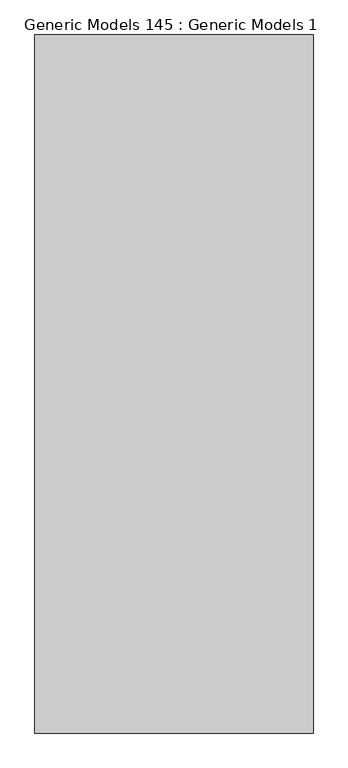
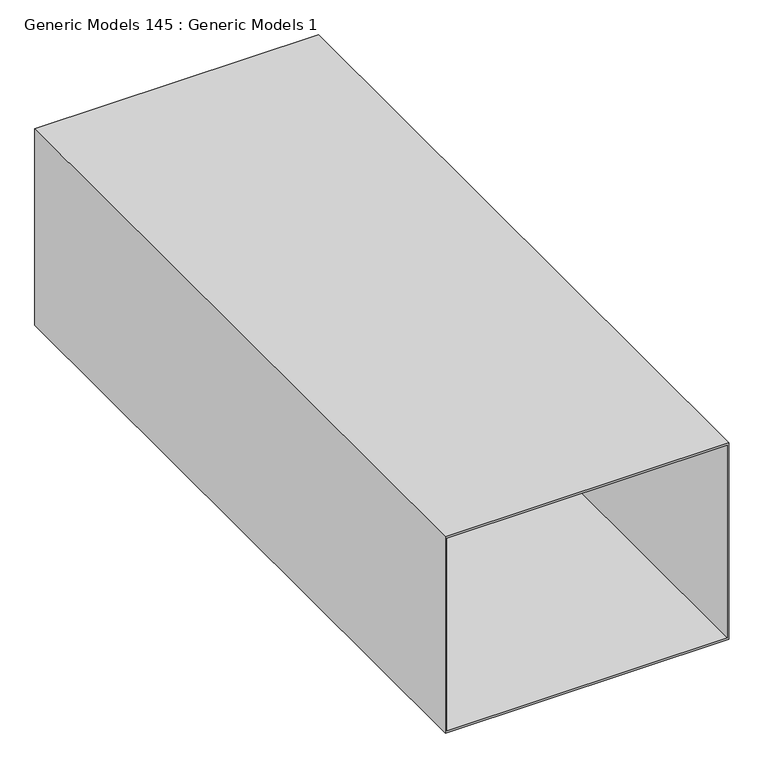
"""IFC4 building model written with IfcOpenShell, lengths in millimetres: proxy geometry, Generic Models 145 : Generic Models 1."""

from ifc_helpers import new_model, si_unit, frame, origin, place, context, project, spatial, polyline, outline, extrude, source, transform, mapped, element, save


def generic_models_145_generic_models_1_d31512ee(model_context):
    return source(origin(), model_context, "Body", "SweptSolid", [
        extrude(outline(polyline([(2028.825, 50664.9319345), (2028.825, 51151.5547769), (2384.425, 51151.5547769), (2384.425, 50664.9319345), (2028.825, 50664.9319345)]), holes=[polyline([(2381.25, 51148.3797769), (2032.0, 51148.3797769), (2032.0, 50668.1069345), (2381.25, 50668.1069345), (2381.25, 51148.3797769)])]), frame((0.0, 0.0, 0.0), z_axis=(0.0, 1.0, 0.0), x_axis=(0.0, 0.0, 1.0)), (0.0, 0.0, 1.0), 1219.2),
    ])


if __name__ == "__main__":
    model = new_model("IFC4")
    model_context = context("Model", 3, world=origin())
    ifc_project = project(units=[si_unit("LENGTHUNIT", "METRE", prefix="MILLI")], contexts=[model_context])
    site = spatial("IfcSite", under=ifc_project)
    building = spatial("IfcBuilding", under=site)
    placement = place(None, origin())
    generic_models_145_generic_models_1_shape = generic_models_145_generic_models_1_d31512ee(model_context)
    element("IfcBuildingElementProxy", 1, Name="Generic Models 145 : Generic Models 1", ObjectType="Generic Models 145 : Generic Models 1", at=placement, inside=building, context=model_context, shape_type="MappedRepresentation", body=[
        mapped(generic_models_145_generic_models_1_shape, transform((0.0, 0.0, 0.0), x_axis=(1.0, 0.0, 0.0), y_axis=(0.0, 1.0, 0.0), z_axis=(0.0, 0.0, 1.0))),
    ])
    save(model, "model.ifc")

# Revit data of these elements
# Element 1 (IfcBuildingElementProxy, "Generic Models 145 : Generic Models 1")
#   Materials on its faces: "EXISTING DUCT"
# Materials
#   "EXISTING DUCT": class "Generic", colour RGB 120 120 120, transparency 0, Cost = 0
